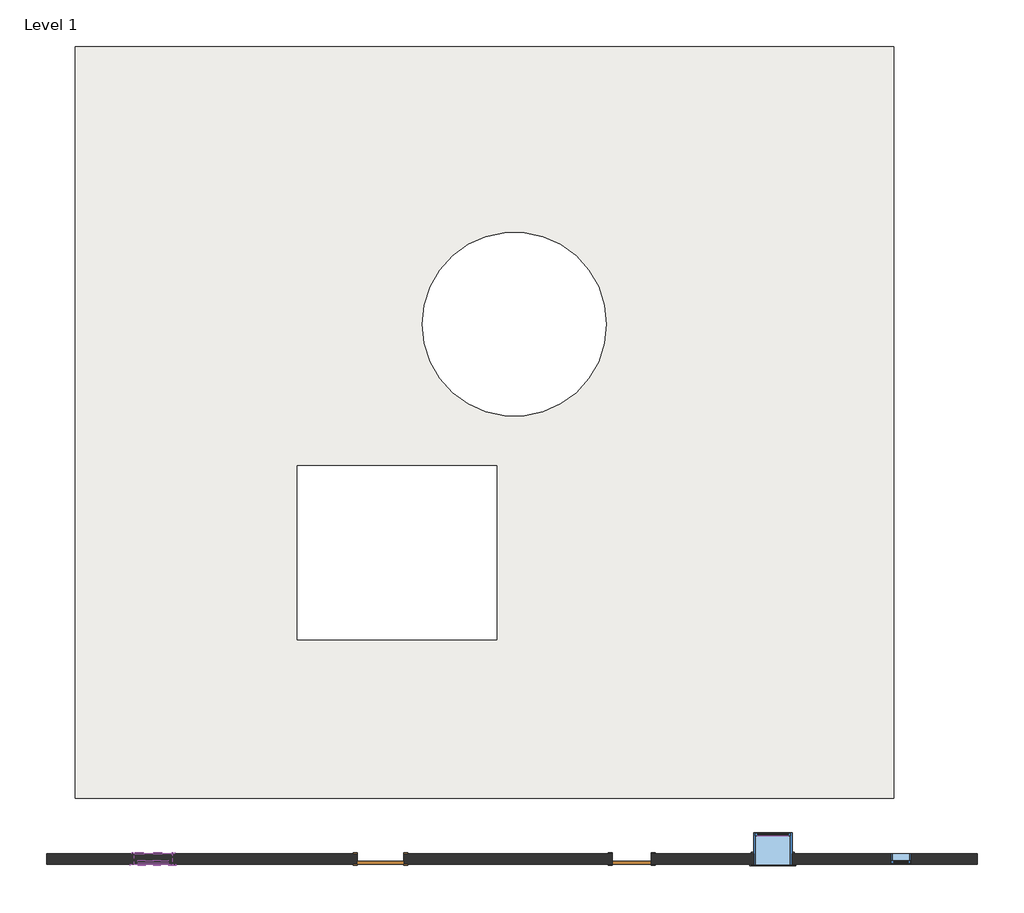
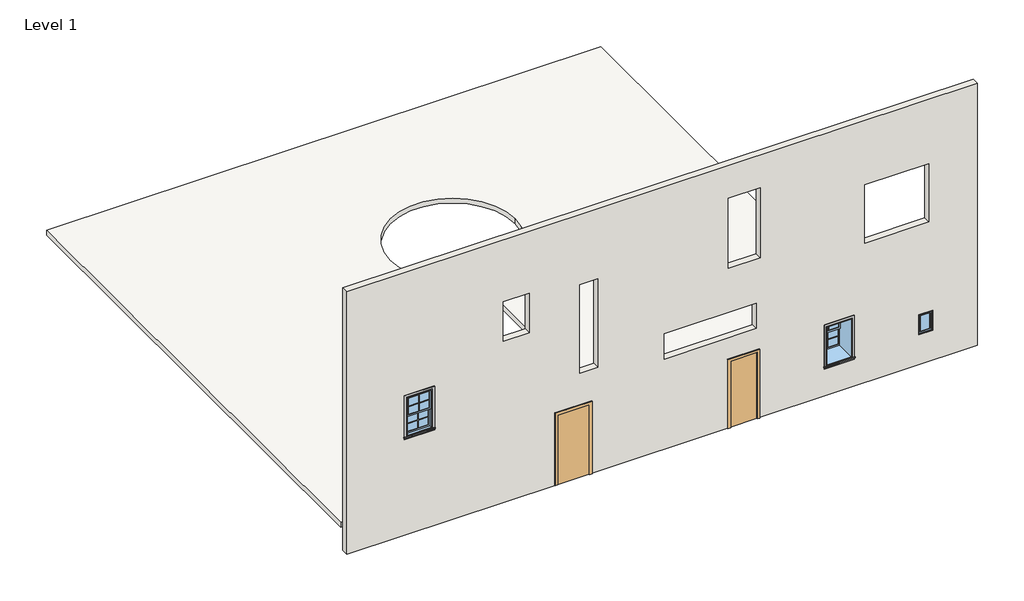
# One storey: 8 proxies, 3 windows, 2 doors, 1 slab, 1 wall.
"""IFC4 building model written with IfcOpenShell, lengths in millimetres."""

import ifcopenshell
import ifcopenshell.guid

model = None  # the IFC model being written
_history = None  # IfcOwnerHistory: only IFC2X3 demands one
_inside = {}  # id of a spatial element -> (the spatial element, [elements in it])
_under = {}  # id of a project, library or spatial element -> (it, [spatial elements below it])
_declared = {}  # id of a project -> (the project, [libraries it declares])
_typed = {}  # id of a type object -> (the type object, [elements of that type])
_made_of = {}  # id of a material, layer set ... -> (it, [elements and type objects made of it])


def new_model(schema):
    """Start an empty IFC model of exactly this schema.

    Asked for "IFC4X3", IfcOpenShell would pick the latest addendum, in which some entities
    have other attributes; the version numbers below select the first issue.
    IFC2X3 requires an IfcOwnerHistory on every rooted entity: one is made here for all.
    """
    global model, _history
    if schema == "IFC4X3":
        model = ifcopenshell.file(schema_version=(4, 3, 0, 0))
    else:
        model = ifcopenshell.file(schema=schema)
    _inside.clear()
    _under.clear()
    _declared.clear()
    _typed.clear()
    _made_of.clear()
    _history = None
    if model.schema == "IFC2X3":
        org = make("IfcOrganization", Name="unknown")
        user = make(
            "IfcPersonAndOrganization",
            ThePerson=make("IfcPerson", FamilyName="unknown"),
            TheOrganization=org,
        )
        app = make(
            "IfcApplication",
            ApplicationDeveloper=org,
            Version="unknown",
            ApplicationFullName="unknown",
            ApplicationIdentifier="unknown",
        )
        _history = make(
            "IfcOwnerHistory",
            OwningUser=user,
            OwningApplication=app,
            ChangeAction="ADDED",
            CreationDate=0,
        )
    return model


def make(cls, **values):
    """One entity of the class cls with the attributes given. An attribute that is None is left unset."""
    return model.create_entity(
        cls, **{name: value for name, value in values.items() if value is not None}
    )


def rooted(cls, **values):
    """An entity with a GlobalId (a new one), such as an element, a storey or a relation."""
    return make(cls, GlobalId=ifcopenshell.guid.new(), OwnerHistory=_history, **values)


def si_unit(unit_type, name, prefix=None):
    """IfcSIUnit, for example si_unit("LENGTHUNIT", "METRE", prefix="MILLI")."""
    return make("IfcSIUnit", UnitType=unit_type, Prefix=prefix, Name=name)


def assignment(units):
    """IfcUnitAssignment: the units of a project."""
    return None if units is None else make("IfcUnitAssignment", Units=units)


def point(xyz):
    """IfcCartesianPoint."""
    return None if xyz is None else make("IfcCartesianPoint", Coordinates=xyz)


def direction(xyz):
    """IfcDirection."""
    return None if xyz is None else make("IfcDirection", DirectionRatios=xyz)


def frame(location, z_axis=None, x_axis=None):
    """IfcAxis2Placement3D, a coordinate frame: its origin and axes. An axis left out is left unset."""
    return make(
        "IfcAxis2Placement3D",
        Location=point(location),
        Axis=direction(z_axis),
        RefDirection=direction(x_axis),
    )


def frame_2d(location, x_axis=None):
    """IfcAxis2Placement2D, a coordinate frame in the plane: its origin and x axis."""
    return make(
        "IfcAxis2Placement2D", Location=point(location), RefDirection=direction(x_axis)
    )


def origin():
    """The frame at (0, 0, 0) with its axes left unset."""
    return frame((0.0, 0.0, 0.0))


def origin_with_axes():
    """The frame at (0, 0, 0) with the z axis (0, 0, 1) and the x axis (1, 0, 0) written out."""
    return frame((0.0, 0.0, 0.0), z_axis=(0.0, 0.0, 1.0), x_axis=(1.0, 0.0, 0.0))


def place(relative_to, where):
    """IfcLocalPlacement: puts the frame where relative to a parent placement (None: the world)."""
    return make(
        "IfcLocalPlacement", PlacementRelTo=relative_to, RelativePlacement=where
    )


def context(
    kind, dimensions, precision=None, world=None, true_north=None, identifier=None
):
    """IfcGeometricRepresentationContext, for example the 3D "Model" context."""
    return make(
        "IfcGeometricRepresentationContext",
        ContextIdentifier=identifier,
        ContextType=kind,
        CoordinateSpaceDimension=dimensions,
        Precision=precision,
        WorldCoordinateSystem=world,
        TrueNorth=true_north,
    )


def project(units=None, contexts=None):
    """IfcProject with its units and contexts."""
    return rooted(
        "IfcProject",
        Name="project",
        RepresentationContexts=contexts,
        UnitsInContext=assignment(units),
    )


def spatial(cls, under=None, at=None, **own):
    """A site, building, storey or space (cls), placed at a placement, below another one or the project."""
    s = rooted(cls, ObjectPlacement=at, **own)
    if under is not None:
        _under.setdefault(under.id(), (under, []))[1].append(s)
    return s


def polyline(points):
    """IfcPolyline through the points."""
    return make("IfcPolyline", Points=[point(p) for p in points])


def circle_curve(where, radius):
    """IfcCircle in the frame where."""
    return make("IfcCircle", Position=where, Radius=radius)


def trimmed(basis, trim1, trim2, sense, master):
    """IfcTrimmedCurve: the piece of a basis curve between two trims."""
    return make(
        "IfcTrimmedCurve",
        BasisCurve=basis,
        Trim1=trim1,
        Trim2=trim2,
        SenseAgreement=sense,
        MasterRepresentation=master,
    )


def segment(curve, same_sense, transition):
    """IfcCompositeCurveSegment."""
    return make(
        "IfcCompositeCurveSegment",
        Transition=transition,
        SameSense=same_sense,
        ParentCurve=curve,
    )


def composite_curve(segments, self_intersect=None):
    """IfcCompositeCurve: segments joined end to end."""
    return make("IfcCompositeCurve", Segments=segments, SelfIntersect=self_intersect)


def outline(outer, holes=None, kind="AREA"):
    """IfcArbitraryClosedProfileDef: a profile drawn as a closed curve; with holes, ...WithVoids."""
    if holes is None:
        return make("IfcArbitraryClosedProfileDef", ProfileType=kind, OuterCurve=outer)
    return make(
        "IfcArbitraryProfileDefWithVoids",
        ProfileType=kind,
        OuterCurve=outer,
        InnerCurves=holes,
    )


def extrude(swept, where, along, depth):
    """IfcExtrudedAreaSolid: the profile swept, set in the frame where, extruded along a direction by depth."""
    return make(
        "IfcExtrudedAreaSolid",
        SweptArea=swept,
        Position=where,
        ExtrudedDirection=direction(along),
        Depth=depth,
    )


def shape(context_of_items, identifier, shape_type, items):
    """IfcShapeRepresentation: the items that make up one representation, for example the "Body"."""
    return make(
        "IfcShapeRepresentation",
        ContextOfItems=context_of_items,
        RepresentationIdentifier=identifier,
        RepresentationType=shape_type,
        Items=items,
    )


def source(mapping_origin, context_of_items, identifier, shape_type, items):
    """IfcRepresentationMap: a shape defined once, which mapped items show again and again."""
    return make(
        "IfcRepresentationMap",
        MappingOrigin=mapping_origin,
        MappedRepresentation=shape(context_of_items, identifier, shape_type, items),
    )


def transform(
    local_origin,
    x_axis=None,
    y_axis=None,
    z_axis=None,
    scale=None,
    scale2=None,
    scale3=None,
    uniform=True,
):
    """IfcCartesianTransformationOperator3D, or its non-uniform kind. x_axis, y_axis, z_axis: its Axis1, 2, 3."""
    if uniform:
        return make(
            "IfcCartesianTransformationOperator3D",
            Axis1=direction(x_axis),
            Axis2=direction(y_axis),
            LocalOrigin=point(local_origin),
            Scale=scale,
            Axis3=direction(z_axis),
        )
    return make(
        "IfcCartesianTransformationOperator3DnonUniform",
        Axis1=direction(x_axis),
        Axis2=direction(y_axis),
        LocalOrigin=point(local_origin),
        Scale=scale,
        Axis3=direction(z_axis),
        Scale2=scale2,
        Scale3=scale3,
    )


def mapped(mapping_source, mapping_target):
    """IfcMappedItem: shows the shape of a source again, moved by a transform."""
    return make(
        "IfcMappedItem", MappingSource=mapping_source, MappingTarget=mapping_target
    )


def made_of(thing, what):
    """Note that an element or type object is made of a material, layer set ...; save() writes the relation."""
    if what is not None:
        _made_of.setdefault(what.id(), (what, []))[1].append(thing)
    return thing


def element(
    cls,
    number,
    at=None,
    inside=None,
    cuts=None,
    type_object=None,
    material=None,
    context=None,
    identifier="Body",
    shape_type=None,
    held_by="IfcProductDefinitionShape",
    body=None,
    shapes=None,
    **own,
):
    """One element of the class cls, such as IfcWall. Its Tag is "e" and its number.

    at: its placement. inside: the storey or other place that contains it. cuts: it is an
    opening in that element (IfcRelVoidsElement). A single representation is given by context,
    identifier, shape_type and body (its items); several are given by shapes. held_by: the class
    of the entity that holds the representations. save() writes the other relations.
    """
    e = rooted(cls, Tag="e%d" % number, ObjectPlacement=at, **own)
    if body is not None:
        shapes = [shape(context, identifier, shape_type, body)]
    if shapes is not None:
        e.Representation = make(held_by, Representations=shapes)
    if inside is not None:
        _inside.setdefault(inside.id(), (inside, []))[1].append(e)
    if cuts is not None:
        rooted(
            "IfcRelVoidsElement", RelatingBuildingElement=cuts, RelatedOpeningElement=e
        )
    if type_object is not None:
        _typed.setdefault(type_object.id(), (type_object, []))[1].append(e)
    return made_of(e, material)


def aggregate(whole, parts):
    """IfcRelAggregates: a whole, such as a stair, and the parts it consists of."""
    return rooted("IfcRelAggregates", RelatingObject=whole, RelatedObjects=parts)


def save(model, path):
    """Write the relations noted so far, then the file.

    IfcRelAggregates (storeys below a building ...), IfcRelContainedInSpatialStructure (elements
    in a storey), IfcRelDefinesByType, IfcRelAssociatesMaterial and IfcRelDeclares: one each for
    every whole, place, type object, material and project.
    """
    for whole, parts in _under.values():
        aggregate(whole, parts)
    for where, things in _inside.values():
        rooted(
            "IfcRelContainedInSpatialStructure",
            RelatedElements=things,
            RelatingStructure=where,
        )
    for kind, things in _typed.values():
        rooted("IfcRelDefinesByType", RelatedObjects=things, RelatingType=kind)
    for what, things in _made_of.values():
        rooted("IfcRelAssociatesMaterial", RelatedObjects=things, RelatingMaterial=what)
    for by, libraries in _declared.values():
        rooted("IfcRelDeclares", RelatingContext=by, RelatedDefinitions=libraries)
    model.write(path)


def m_muntin_pattern_2x2_m_muntin_pattern_2x2_aaec3afb(model_context):
    return source(origin(), model_context, "Body", "SweptSolid", [
        extrude(outline(polyline([(257.1375, -6.35), (257.1375, -298.8), (244.4375, -298.8), (244.4375, -6.35), (0.0, -6.35), (0.0, 6.35), (244.4375, 6.35), (244.4375, 298.8), (257.1375, 298.8), (257.1375, 6.35), (501.575, 6.35), (501.575, -6.35), (257.1375, -6.35)])), frame((0.0, 9.525, 0.0), z_axis=(0.0, 1.0, 0.0), x_axis=(0.0, 0.0, 1.0)), (0.0, 0.0, 1.0), 12.7),
        extrude(outline(polyline([(257.1375, -6.35), (257.1375, -298.8), (244.4375, -298.8), (244.4375, -6.35), (0.0, -6.35), (0.0, 6.35), (244.4375, 6.35), (244.4375, 298.8), (257.1375, 298.8), (257.1375, 6.35), (501.575, 6.35), (501.575, -6.35), (257.1375, -6.35)])), frame((0.0, -22.225, 0.0), z_axis=(0.0, 1.0, 0.0), x_axis=(0.0, 0.0, 1.0)), (0.0, 0.0, 1.0), 12.7),
    ])


def m_trim_window_exterior_flat_with_sill_e7ff6350(model_context):
    return source(origin(), model_context, "Body", "SweptSolid", [
        extrude(outline(polyline([(435.0, -1220.4323709), (435.0, -1280.4323709), (-435.0, -1280.4323709), (-435.0, -1220.4323709), (435.0, -1220.4323709)])), origin_with_axes(), (0.0, 0.0, 1.0), 19.05),
        extrude(outline(polyline([(-1230.0, 38.1), (-1202.4580645, 38.1), (-1200.0, 19.05), (-1200.0, 0.0), (-1220.4323709, 0.0), (-1220.4323709, 19.05), (-1230.0, 19.05), (-1230.0, 38.1)])), frame((-447.7, 0.0, 0.0), z_axis=(1.0, 0.0, 0.0), x_axis=(0.0, 1.0, 0.0)), (0.0, 0.0, 1.0), 895.4),
        extrude(outline(polyline([(-435.0, 60.0), (435.0, 60.0), (435.0, -1200.0), (375.0, -1200.0), (375.0, 0.0), (-375.0, 0.0), (-375.0, -1200.0), (-435.0, -1200.0), (-435.0, 60.0)])), origin_with_axes(), (0.0, 0.0, 1.0), 19.05),
    ])


def m_trim_window_interior_flat_picture_frame_31bd2320(model_context):
    return source(origin(), model_context, "Body", "SweptSolid", [
        extrude(outline(polyline([(422.3, 47.3), (422.3, -1247.3), (-422.3, -1247.3), (-422.3, 47.3), (422.3, 47.3)]), holes=[polyline([(362.3, -12.7), (-362.3, -12.7), (-362.3, -1187.3), (362.3, -1187.3), (362.3, -12.7)])]), origin_with_axes(), (0.0, 0.0, 1.0), 30.0),
    ])


def m_single_flush_0762_x_2032mm_0c256fab(model_context):
    return source(origin(), model_context, "Body", "SweptSolid", [
        extrude(outline(polyline([(2108.0, -457.0), (0.0, -457.0), (0.0, -381.0), (2032.0, -381.0), (2032.0, 381.0), (0.0, 381.0), (0.0, 457.0), (2108.0, 457.0), (2108.0, -457.0)])), frame((0.0, 100.0, 0.0), z_axis=(0.0, 1.0, 0.0), x_axis=(0.0, 0.0, 1.0)), (0.0, 0.0, 1.0), 25.0),
        extrude(outline(polyline([(2108.0, 457.0), (2108.0, -457.0), (0.0, -457.0), (0.0, -381.0), (2032.0, -381.0), (2032.0, 381.0), (0.0, 381.0), (0.0, 457.0), (2108.0, 457.0)])), frame((0.0, -125.0, 0.0), z_axis=(0.0, 1.0, 0.0), x_axis=(0.0, 0.0, 1.0)), (0.0, 0.0, 1.0), 25.0),
        extrude(outline(polyline([(381.0, 49.0), (-381.0, 49.0), (-381.0, 100.0), (381.0, 100.0), (381.0, 49.0)])), origin_with_axes(), (0.0, 0.0, 1.0), 2032.0),
    ])


def m_single_flush_0915_x_2134mm_727434cd(model_context):
    return source(origin(), model_context, "Body", "SweptSolid", [
        extrude(outline(polyline([(2210.0, -533.5), (0.0, -533.5), (0.0, -457.5), (2134.0, -457.5), (2134.0, 457.5), (0.0, 457.5), (0.0, 533.5), (2210.0, 533.5), (2210.0, -533.5)])), frame((0.0, -125.0, 0.0), z_axis=(0.0, 1.0, 0.0), x_axis=(0.0, 0.0, 1.0)), (0.0, 0.0, 1.0), 25.0),
        extrude(outline(polyline([(2210.0, 533.5), (2210.0, -533.5), (0.0, -533.5), (0.0, -457.5), (2134.0, -457.5), (2134.0, 457.5), (0.0, 457.5), (0.0, 533.5), (2210.0, 533.5)])), frame((0.0, 100.0, 0.0), z_axis=(0.0, 1.0, 0.0), x_axis=(0.0, 0.0, 1.0)), (0.0, 0.0, 1.0), 25.0),
        extrude(outline(polyline([(457.5, -49.0), (457.5, -100.0), (-457.5, -100.0), (-457.5, -49.0), (457.5, -49.0)])), origin_with_axes(), (0.0, 0.0, 1.0), 2134.0),
    ])


def m_fixed_0406_x_0610mm_8205b201(model_context):
    return source(origin(), model_context, "Body", "SweptSolid", [
        extrude(outline(polyline([(-140.0, 78.0), (140.0, 78.0), (140.0, 66.0), (-140.0, 66.0), (-140.0, 78.0)])), frame((0.0, 0.0, 978.0), z_axis=(0.0, 0.0, 1.0), x_axis=(1.0, 0.0, 0.0)), (0.0, 0.0, 1.0), 484.0),
        extrude(outline(polyline([(1506.0, -184.0), (934.0, -184.0), (934.0, 184.0), (1506.0, 184.0), (1506.0, -184.0)]), holes=[polyline([(1462.0, -140.0), (1462.0, 140.0), (978.0, 140.0), (978.0, -140.0), (1462.0, -140.0)])]), frame((0.0, 50.0, 0.0), z_axis=(0.0, 1.0, 0.0), x_axis=(0.0, 0.0, 1.0)), (0.0, 0.0, 1.0), 44.0),
        extrude(outline(polyline([(1525.0, -203.0), (915.0, -203.0), (915.0, 203.0), (1525.0, 203.0), (1525.0, -203.0)]), holes=[polyline([(1506.0, -184.0), (1506.0, 184.0), (934.0, 184.0), (934.0, -184.0), (1506.0, -184.0)])]), frame((0.0, 50.0, 0.0), z_axis=(0.0, 1.0, 0.0), x_axis=(0.0, 0.0, 1.0)), (0.0, 0.0, 1.0), 63.0),
        extrude(outline(polyline([(1525.0, -203.0), (915.0, -203.0), (915.0, 203.0), (1525.0, 203.0), (1525.0, -203.0)]), holes=[polyline([(1493.0, -171.0), (1493.0, 171.0), (947.0, 171.0), (947.0, -171.0), (1493.0, -171.0)])]), frame((0.0, -87.0, 0.0), z_axis=(0.0, 1.0, 0.0), x_axis=(0.0, 0.0, 1.0)), (0.0, 0.0, 1.0), 137.0),
    ])


def m_window_double_hung_750_x_1200mm_41070976(model_context):
    return source(origin(), model_context, "Body", "SweptSolid", [
        extrude(outline(polyline([(298.8, 30.15), (298.8, 23.8), (-298.8, 23.8), (-298.8, 30.15), (298.8, 30.15)])), frame((0.0, 0.0, 990.6), z_axis=(0.0, 0.0, 1.0), x_axis=(1.0, 0.0, 0.0)), (0.0, 0.0, 1.0), 501.575),
        extrude(outline(polyline([(-298.8, 17.45), (298.8, 17.45), (298.8, 11.1), (-298.8, 11.1), (-298.8, 17.45)])), frame((0.0, 0.0, 990.6), z_axis=(0.0, 0.0, 1.0), x_axis=(1.0, 0.0, 0.0)), (0.0, 0.0, 1.0), 501.575),
        extrude(outline(polyline([(298.8, 74.6), (298.8, 68.25), (-298.8, 68.25), (-298.8, 74.6), (298.8, 74.6)])), frame((0.0, 0.0, 1536.625), z_axis=(0.0, 0.0, 1.0), x_axis=(1.0, 0.0, 0.0)), (0.0, 0.0, 1.0), 501.575),
        extrude(outline(polyline([(-298.8, 61.9), (298.8, 61.9), (298.8, 55.55), (-298.8, 55.55), (-298.8, 61.9)])), frame((0.0, 0.0, 1536.625), z_axis=(0.0, 0.0, 1.0), x_axis=(1.0, 0.0, 0.0)), (0.0, 0.0, 1.0), 501.575),
        extrude(outline(polyline([(1536.625, -343.25), (946.15, -343.25), (946.15, 343.25), (1536.625, 343.25), (1536.625, -343.25)]), holes=[polyline([(1492.175, 298.8), (990.6, 298.8), (990.6, -298.8), (1492.175, -298.8), (1492.175, 298.8)])]), frame((0.0, -1.6, 0.0), z_axis=(0.0, 1.0, 0.0), x_axis=(0.0, 0.0, 1.0)), (0.0, 0.0, 1.0), 44.45),
        extrude(outline(polyline([(2082.65, -343.25), (1492.175, -343.25), (1492.175, 343.25), (2082.65, 343.25), (2082.65, -343.25)]), holes=[polyline([(2038.2, 298.8), (1536.625, 298.8), (1536.625, -298.8), (2038.2, -298.8), (2038.2, 298.8)])]), frame((0.0, 42.85, 0.0), z_axis=(0.0, 1.0, 0.0), x_axis=(0.0, 0.0, 1.0)), (0.0, 0.0, 1.0), 44.45),
        extrude(outline(polyline([(2114.4, -375.0), (914.4, -375.0), (914.4, 375.0), (2114.4, 375.0), (2114.4, -375.0)]), holes=[polyline([(2082.65, 343.25), (946.15, 343.25), (946.15, -343.25), (2082.65, -343.25), (2082.65, 343.25)])]), frame((0.0, -14.3, 0.0), z_axis=(0.0, 1.0, 0.0), x_axis=(0.0, 0.0, 1.0)), (0.0, 0.0, 1.0), 133.35),
        extrude(outline(polyline([(2114.4, 375.0), (2114.4, -375.0), (914.4, -375.0), (914.4, 375.0), (2114.4, 375.0)]), holes=[polyline([(2095.35, 355.95), (933.45, 355.95), (933.45, -355.95), (2095.35, -355.95), (2095.35, 355.95)])]), frame((0.0, -100.0, 0.0), z_axis=(0.0, 1.0, 0.0), x_axis=(0.0, 0.0, 1.0)), (0.0, 0.0, 1.0), 85.7),
    ])


def m_window_double_hung_750_x_1200mm_e21ea802(model_context):
    return source(origin(), model_context, "Body", "SweptSolid", [
        extrude(outline(polyline([(298.8, -469.85), (298.8, -476.2), (-298.8, -476.2), (-298.8, -469.85), (298.8, -469.85)])), frame((0.0, 0.0, 990.6), z_axis=(0.0, 0.0, 1.0), x_axis=(1.0, 0.0, 0.0)), (0.0, 0.0, 1.0), 501.575),
        extrude(outline(polyline([(-298.8, -482.55), (298.8, -482.55), (298.8, -488.9), (-298.8, -488.9), (-298.8, -482.55)])), frame((0.0, 0.0, 990.6), z_axis=(0.0, 0.0, 1.0), x_axis=(1.0, 0.0, 0.0)), (0.0, 0.0, 1.0), 501.575),
        extrude(outline(polyline([(298.8, -425.4), (298.8, -431.75), (-298.8, -431.75), (-298.8, -425.4), (298.8, -425.4)])), frame((0.0, 0.0, 1536.625), z_axis=(0.0, 0.0, 1.0), x_axis=(1.0, 0.0, 0.0)), (0.0, 0.0, 1.0), 501.575),
        extrude(outline(polyline([(-298.8, -438.1), (298.8, -438.1), (298.8, -444.45), (-298.8, -444.45), (-298.8, -438.1)])), frame((0.0, 0.0, 1536.625), z_axis=(0.0, 0.0, 1.0), x_axis=(1.0, 0.0, 0.0)), (0.0, 0.0, 1.0), 501.575),
        extrude(outline(polyline([(1536.625, -343.25), (946.15, -343.25), (946.15, 343.25), (1536.625, 343.25), (1536.625, -343.25)]), holes=[polyline([(1492.175, 298.8), (990.6, 298.8), (990.6, -298.8), (1492.175, -298.8), (1492.175, 298.8)])]), frame((0.0, -501.6, 0.0), z_axis=(0.0, 1.0, 0.0), x_axis=(0.0, 0.0, 1.0)), (0.0, 0.0, 1.0), 44.45),
        extrude(outline(polyline([(2082.65, -343.25), (1492.175, -343.25), (1492.175, 343.25), (2082.65, 343.25), (2082.65, -343.25)]), holes=[polyline([(2038.2, 298.8), (1536.625, 298.8), (1536.625, -298.8), (2038.2, -298.8), (2038.2, 298.8)])]), frame((0.0, -457.15, 0.0), z_axis=(0.0, 1.0, 0.0), x_axis=(0.0, 0.0, 1.0)), (0.0, 0.0, 1.0), 44.45),
        extrude(outline(polyline([(2114.4, -375.0), (914.4, -375.0), (914.4, 375.0), (2114.4, 375.0), (2114.4, -375.0)]), holes=[polyline([(2082.65, 343.25), (946.15, 343.25), (946.15, -343.25), (2082.65, -343.25), (2082.65, 343.25)])]), frame((0.0, -514.3, 0.0), z_axis=(0.0, 1.0, 0.0), x_axis=(0.0, 0.0, 1.0)), (0.0, 0.0, 1.0), 633.35),
    ])


model = new_model("IFC4")

# Units and contexts
model_context = context("Model", 3, world=origin())
ifc_project = project(units=[si_unit("LENGTHUNIT", "METRE", prefix="MILLI")], contexts=[model_context])

# Site, building, storey
site = spatial("IfcSite", under=ifc_project)
building = spatial("IfcBuilding", under=site)
storey = spatial("IfcBuildingStorey", under=building, Name="Level 1", Elevation=0.0)

# Proxies
placement = place(None, origin())
m_muntin_pattern_2x2_m_muntin_pattern_2x2_shape = m_muntin_pattern_2x2_m_muntin_pattern_2x2_aaec3afb(model_context)
element("IfcBuildingElementProxy", 1, Name="M_Muntin Pattern_2x2 : M_Muntin Pattern_2x2", ObjectType="M_Muntin Pattern_2x2 : M_Muntin Pattern_2x2", at=placement, inside=storey, context=model_context, shape_type="MappedRepresentation", body=[
    mapped(m_muntin_pattern_2x2_m_muntin_pattern_2x2_shape, transform((-9517.9287267, -12044.9889904, 3622.225), x_axis=(-1.0, 0.0, 0.0), y_axis=(0.0, -1.0, 0.0), z_axis=(0.0, 0.0, 1.0))),
])
element("IfcBuildingElementProxy", 2, Name="M_Muntin Pattern_2x2 : M_Muntin Pattern_2x2", ObjectType="M_Muntin Pattern_2x2 : M_Muntin Pattern_2x2", at=placement, inside=storey, context=model_context, shape_type="MappedRepresentation", body=[
    mapped(m_muntin_pattern_2x2_m_muntin_pattern_2x2_shape, transform((-9517.9287267, -12000.5389904, 3076.2), x_axis=(-1.0, 0.0, 0.0), y_axis=(0.0, -1.0, 0.0), z_axis=(0.0, 0.0, 1.0))),
])
element("IfcBuildingElementProxy", 3, Name="M_Muntin Pattern_2x2 : M_Muntin Pattern_2x2", ObjectType="M_Muntin Pattern_2x2 : M_Muntin Pattern_2x2", at=placement, inside=storey, context=model_context, shape_type="MappedRepresentation", body=[
    mapped(m_muntin_pattern_2x2_m_muntin_pattern_2x2_shape, transform((2597.0712733, -11544.9889904, 1536.625), x_axis=(-1.0, 0.0, 0.0), y_axis=(0.0, -1.0, 0.0), z_axis=(0.0, 0.0, 1.0))),
])
element("IfcBuildingElementProxy", 4, Name="M_Muntin Pattern_2x2 : M_Muntin Pattern_2x2", ObjectType="M_Muntin Pattern_2x2 : M_Muntin Pattern_2x2", at=placement, inside=storey, context=model_context, shape_type="MappedRepresentation", body=[
    mapped(m_muntin_pattern_2x2_m_muntin_pattern_2x2_shape, transform((2597.0712733, -11500.5389904, 990.6), x_axis=(-1.0, 0.0, 0.0), y_axis=(0.0, -1.0, 0.0), z_axis=(0.0, 0.0, 1.0))),
])
m_trim_window_exterior_flat_with_sill_shape = m_trim_window_exterior_flat_with_sill_e7ff6350(model_context)
element("IfcBuildingElementProxy", 5, Name="M_Trim-Window-Exterior-Flat : with Sill", ObjectType="M_Trim-Window-Exterior-Flat : with Sill", at=placement, inside=storey, context=model_context, shape_type="MappedRepresentation", body=[
    mapped(m_trim_window_exterior_flat_with_sill_shape, transform((-9517.9287267, -12079.9139904, 4200.0), x_axis=(1.0, 0.0, 0.0), y_axis=(0.0, 0.0, 1.0), z_axis=(0.0, -1.0, 0.0))),
])
element("IfcBuildingElementProxy", 6, Name="M_Trim-Window-Exterior-Flat : with Sill", ObjectType="M_Trim-Window-Exterior-Flat : with Sill", at=placement, inside=storey, context=model_context, shape_type="MappedRepresentation", body=[
    mapped(m_trim_window_exterior_flat_with_sill_shape, transform((2597.0712733, -12079.9139904, 2114.4), x_axis=(1.0, 0.0, 0.0), y_axis=(0.0, 0.0, 1.0), z_axis=(0.0, -1.0, 0.0))),
])
m_trim_window_interior_flat_picture_frame_shape = m_trim_window_interior_flat_picture_frame_31bd2320(model_context)
element("IfcBuildingElementProxy", 7, Name="M_Trim-Window-Interior-Flat : Picture Frame", ObjectType="M_Trim-Window-Interior-Flat : Picture Frame", at=placement, inside=storey, context=model_context, shape_type="MappedRepresentation", body=[
    mapped(m_trim_window_interior_flat_picture_frame_shape, transform((-9517.9287267, -11879.9139904, 4200.0), x_axis=(-1.0, 0.0, 0.0), y_axis=(0.0, 0.0, 1.0), z_axis=(0.0, 1.0, 0.0))),
])
element("IfcBuildingElementProxy", 8, Name="M_Trim-Window-Interior-Flat : Picture Frame", ObjectType="M_Trim-Window-Interior-Flat : Picture Frame", at=placement, inside=storey, context=model_context, shape_type="MappedRepresentation", body=[
    mapped(m_trim_window_interior_flat_picture_frame_shape, transform((2597.0712733, -11879.9139904, 2114.4), x_axis=(-1.0, 0.0, 0.0), y_axis=(0.0, 0.0, 1.0), z_axis=(0.0, 1.0, 0.0))),
])

# Doors
m_single_flush_0762_x_2032mm_shape = m_single_flush_0762_x_2032mm_0c256fab(model_context)
element("IfcDoor", 9, ObjectType="M_Single-Flush : 0762 x 2032mm", at=placement, inside=storey, context=model_context, shape_type="MappedRepresentation", body=[
    mapped(m_single_flush_0762_x_2032mm_shape, transform((-160.4287267, -11979.9139904, 0.0), x_axis=(-1.0, 0.0, 0.0), y_axis=(0.0, -1.0, 0.0), z_axis=(0.0, 0.0, 1.0))),
])
m_single_flush_0915_x_2134mm_shape = m_single_flush_0915_x_2134mm_727434cd(model_context)
element("IfcDoor", 10, ObjectType="M_Single-Flush : 0915 x 2134mm", at=placement, inside=storey, context=model_context, shape_type="MappedRepresentation", body=[
    mapped(m_single_flush_0915_x_2134mm_shape, transform((-5075.4287267, -11979.9139904, 0.0), x_axis=(1.0, 0.0, 0.0), y_axis=(0.0, 1.0, 0.0), z_axis=(0.0, 0.0, 1.0))),
])

# Slab
element("IfcSlab", 11, ObjectType="Generic 150mm", at=placement, inside=storey, context=model_context, shape_type="SweptSolid", body=[
    extrude(outline(polyline([(4955.9656102, -10797.4121597), (-11044.0343898, -10797.4121597), (-11044.0343898, 3902.5878403), (4955.9656102, 3902.5878403), (4955.9656102, -10797.4121597)]), holes=[polyline([(-2803.5612558, -7694.4830059), (-2803.5612558, -4294.4830059), (-6703.5612558, -4294.4830059), (-6703.5612558, -7694.4830059), (-2803.5612558, -7694.4830059)]), composite_curve([segment(trimmed(circle_curve(frame_2d((-2455.6131826, -1525.5713844)), 1800.0), [point((-4255.6131826, -1525.5713844))], [point((-655.6131826, -1525.5713844))], True, "CARTESIAN"), True, "CONTINUOUS"), segment(trimmed(circle_curve(frame_2d((-2455.6131826, -1525.5713844)), 1800.0), [point((-655.6131826, -1525.5713844))], [point((-4255.6131826, -1525.5713844))], True, "CARTESIAN"), True, "CONTINUOUS")], self_intersect=False)]), frame((0.0, 0.0, -150.0), z_axis=(0.0, 0.0, 1.0), x_axis=(1.0, 0.0, 0.0)), (0.0, 0.0, 1.0), 150.0),
])

# Wall
element("IfcWall", 12, ObjectType="Generic - 200mm", at=placement, inside=storey, context=model_context, shape_type="SweptSolid", body=[
    extrude(outline(polyline([(0.0, 6597.0712733), (8000.0, 6597.0712733), (8000.0, -11602.9287267), (0.0, -11602.9287267), (0.0, -5532.9287267), (2134.0, -5532.9287267), (2134.0, -4617.9287267), (0.0, -4617.9287267), (0.0, -541.4287267), (2032.0, -541.4287267), (2032.0, 220.5712733), (0.0, 220.5712733), (0.0, 6597.0712733)]), holes=[polyline([(915.0, 5303.0712733), (915.0, 4897.0712733), (1525.0, 4897.0712733), (1525.0, 5303.0712733), (915.0, 5303.0712733)]), polyline([(2114.4, 2972.0712733), (914.4, 2972.0712733), (914.4, 2222.0712733), (2114.4, 2222.0712733), (2114.4, 2972.0712733)]), polyline([(4200.0, -9142.9287267), (3000.0, -9142.9287267), (3000.0, -9892.9287267), (4200.0, -9892.9287267), (4200.0, -9142.9287267)]), polyline([(6114.4, -6332.9287267), (4914.4, -6332.9287267), (4914.4, -7082.9287267), (6114.4, -7082.9287267), (6114.4, -6332.9287267)]), polyline([(4866.0, -592.9287267), (7000.0, -592.9287267), (7000.0, 322.0712733), (4866.0, 322.0712733), (4866.0, -592.9287267)]), polyline([(5863.7369526, -4875.7403935), (5863.7369526, -4355.210627), (3168.8098281, -4355.210627), (3168.8098281, -4875.7403935), (5863.7369526, -4875.7403935)]), polyline([(3522.0583984, -2446.6014834), (3522.0583984, 213.8839896), (2748.6051294, 213.8839896), (2748.6051294, -2446.6014834), (3522.0583984, -2446.6014834)]), polyline([(6036.9886823, 3337.0625883), (6036.9886823, 5187.8350912), (4260.1064286, 5187.8350912), (4260.1064286, 3337.0625883), (6036.9886823, 3337.0625883)])]), frame((0.0, -12079.9139904, 0.0), z_axis=(0.0, 1.0, 0.0), x_axis=(0.0, 0.0, 1.0)), (0.0, 0.0, 1.0), 200.0),
])

# Windows
m_fixed_0406_x_0610mm_shape = m_fixed_0406_x_0610mm_8205b201(model_context)
element("IfcWindow", 13, ObjectType="M_Fixed : 0406 x 0610mm", at=placement, inside=storey, context=model_context, shape_type="MappedRepresentation", body=[
    mapped(m_fixed_0406_x_0610mm_shape, transform((5100.0712733, -11966.9139904, 0.0), x_axis=(-1.0, 0.0, 0.0), y_axis=(0.0, -1.0, 0.0), z_axis=(0.0, 0.0, 1.0))),
])
m_window_double_hung_750_x_1200mm_shape = m_window_double_hung_750_x_1200mm_41070976(model_context)
element("IfcWindow", 14, ObjectType="M_Window-Double-Hung : 750 x 1200mm", at=placement, inside=storey, context=model_context, shape_type="MappedRepresentation", body=[
    mapped(m_window_double_hung_750_x_1200mm_shape, transform((-9517.9287267, -11979.9139904, 2085.6), x_axis=(-1.0, 0.0, 0.0), y_axis=(0.0, -1.0, 0.0), z_axis=(0.0, 0.0, 1.0))),
])
m_window_double_hung_750_x_1200mm_2_shape = m_window_double_hung_750_x_1200mm_e21ea802(model_context)
element("IfcWindow", 15, ObjectType="M_Window-Double-Hung : 750 x 1200mm", at=placement, inside=storey, context=model_context, shape_type="MappedRepresentation", body=[
    mapped(m_window_double_hung_750_x_1200mm_2_shape, transform((2597.0712733, -11979.9139904, 0.0), x_axis=(-1.0, 0.0, 0.0), y_axis=(0.0, -1.0, 0.0), z_axis=(0.0, 0.0, 1.0))),
])

save(model, "model.ifc")

# Revit data of these elements
# Project information
#   Project Issue Date = "Issue Date"
#   Project Status = "Project Status"
#   Client Name = "Owner"
#   Project Address = "Enter address here"
#   Project Name = "Project Name"
#   Project Number = "0001"
# Type "M_Muntin Pattern_2x2 : M_Muntin Pattern_2x2"
#   Width [instance default] = 1200 mm
#   Thickness = 12.7 mm
#   Height [instance default] = 1200 mm
#   Distance = 19.05 mm
#   Interior Material [instance default] = none
#   Exterior Material [instance default] = none
#   Default Elevation = 0
# Type "M_Trim-Window-Exterior-Flat : with Sill"
#   Trim Width = 60 mm
#   Trim Thickness_Picture Frame = 30 mm
#   Trim Thickness_with Sill = 19.05 mm
#   Sill Thickness = 30 mm
#   Opening Width [instance default] = 600 mm
#   Opening Height [instance default] = 900 mm
#   Default Elevation = 1200 mm
#   Sill = yes
#   Picture Frame = no
#   Trim Material [instance default] = none
# Type "M_Trim-Window-Interior-Flat : Picture Frame"
#   Trim Thickness_Picture Frame = 30 mm
#   Trim Width = 60 mm
#   Trim Thickness_with Sill = 20 mm
#   Sill Thickness = 30 mm
#   Opening Width [instance default] = 600 mm
#   Opening Height [instance default] = 900 mm
#   Default Elevation = 1200 mm
#   Sill = no
#   Picture Frame = yes
#   Trim Material [instance default] = none
# Type "M_Single-Flush : 0762 x 2032mm"
#   Type Mark = "28"
#   Construction Type Id = "MDOOR"
#   Analytic Construction = "Metal"
#   Thickness = 51 mm
#   Thermal Resistance (R) = 0.270117 (m²·K)/W
#   Heat Transfer Coefficient (U) = 3.7021 W/(m²·K)
#   Height = 2032 mm
#   Trim Projection Ext = 25 mm
#   Trim Projection Int = 25 mm
#   Trim Width = 76 mm
#   Width = 762 mm
#   Define Thermal Properties by = 1
#   Define Thermal Properties by = 1
#   Door Material = Door - Panel
#   Frame Material = Door - Frame
#   Visual Light Transmittance = 0
#   Solar Heat Gain Coefficient = 0
#   Function = (empty or 0)
#   Wall Closure = (empty or 0)
# Type "M_Single-Flush : 0915 x 2134mm"
#   Type Mark = "20"
#   Construction Type Id = "MDOOR"
#   Analytic Construction = "Metal"
#   Thickness = 51 mm
#   Thermal Resistance (R) = 0.270117 (m²·K)/W
#   Heat Transfer Coefficient (U) = 3.7021 W/(m²·K)
#   Height = 2134 mm
#   Trim Projection Ext = 25 mm
#   Trim Projection Int = 25 mm
#   Trim Width = 76 mm
#   Width = 915 mm
#   Define Thermal Properties by = 1
#   Define Thermal Properties by = 1
#   Door Material = Door - Panel
#   Frame Material = Door - Frame
#   Visual Light Transmittance = 0
#   Solar Heat Gain Coefficient = 0
#   Function = (empty or 0)
#   Wall Closure = (empty or 0)
# Type "Generic 150mm"
#   Function = 0
#   Layers, outside or top first: 150 mm no material (function 1)
# Type "Generic - 200mm"
#   Layers, outside or top first: 200 mm no material (function 1)
# Type "M_Fixed : 0406 x 0610mm"
#   Type Mark = "10"
#   Construction Type Id = "GSP4R"
#   Analytic Construction = "1/8 in Pilkington single glazing"
#   Visual Light Transmittance = 0.9
#   Thermal Resistance (R) = 0.271106 (m²·K)/W
#   Solar Heat Gain Coefficient = 0.78
#   Heat Transfer Coefficient (U) = 3.6886 W/(m²·K)
#   Height = 610 mm
#   Default Sill Height = 915 mm
#   Width = 406 mm
#   Window Inset = 19 mm
#   Define Thermal Properties by = 1
#   Define Thermal Properties by = 1
#   Frame Exterior Material = Sash
#   Frame Interior Material = Sash
#   Glass Pane Material = Glass
#   Sash = Sash
#   Wall Closure = (empty or 0)
# Type "M_Window-Double-Hung : 750 x 1200mm"
#   Type Mark = "22"
#   Fire Rating = "0.5h"
#   Construction Type Id = "DG-DR"
#   Assembly Code = "B2020100"
#   Analytic Construction = "Double glazing - domestic"
#   Wall Thickness [instance default] = 150 mm
#   Window Inset [instance default] = 0 mm
#   Visual Light Transmittance = 0.81
#   Thermal Resistance (R) = 0.319569 (m²·K)/W
#   Solar Heat Gain Coefficient = 0.76
#   Muntin Width = 597.6 mm
#   Muntin Height = 501.575 mm
#   Interior Wall Closure [instance default] = 35.7 mm
#   Rough Width = 765 mm
#   Rough Height = 1215 mm
#   Frame Extension [instance default] = 31.75 mm
#   Exterior Wall Closure [instance default] = 12.7 mm
#   Extension Jamb [instance default] = 35.7 mm
#   Heat Transfer Coefficient (U) = 3.12929 W/(m²·K)
#   Height = 1200 mm
#   Width = 750 mm
#   Define Thermal Properties by = 1
#   Top Muntin Visibility = yes
#   Indicator Visibility [instance default] = yes
#   Extension Jamb Visibility [instance default] = yes
#   Interior Trim Visibility [instance default] = yes
#   Exterior Trim Visibility [instance default] = yes
#   Define Thermal Properties by = 1
#   Bottom Muntin Visibility = yes
#   Muntin Pattern = M_Muntin Pattern_2x2 : M_Muntin Pattern_2x2
#   Interior Trim Material = Wood - Stained
#   Interior Trim = M_Trim-Window-Interior-Flat : Picture Frame
#   Exterior Trim Material = Clad - White
#   Exterior Trim = M_Trim-Window-Exterior-Flat : with Sill
#   Glass Panel Material = Glass
#   Exterior Frame Material = Clad - White
#   Interior Frame Material = Wood - Stained
#   Wall Closure = (empty or 0)
# Elements 1, 2, 3, 4 (IfcBuildingElementProxy, "M_Muntin Pattern_2x2 : M_Muntin Pattern_2x2")
#   Width = 597.6 mm
#   Height = 501.575 mm
#   Interior Material = Wood - Stained
#   Exterior Material = Clad - White
#   Phase Created = New Construction
#   Materials on its faces: "Clad - White", "Wood - Stained"
# Elements 5, 6 (IfcBuildingElementProxy, "M_Trim-Window-Exterior-Flat : with Sill")
#   Opening Width = 750 mm
#   Opening Height = 1200 mm
#   Trim Material = Clad - White
#   Phase Created = New Construction
#   Materials on its faces: "Clad - White"
# Elements 7, 8 (IfcBuildingElementProxy, "M_Trim-Window-Interior-Flat : Picture Frame")
#   Opening Width = 750 mm
#   Opening Height = 1200 mm
#   Trim Material = Wood - Stained
#   Phase Created = New Construction
#   Materials on its faces: "Wood - Stained"
# Element 9 (IfcDoor, "M_Single-Flush : 0762 x 2032mm")
#   Phase Created = New Construction
#   Materials on its faces: "Door - Frame", "Door - Panel"
# Element 10 (IfcDoor, "M_Single-Flush : 0915 x 2134mm")
#   Phase Created = New Construction
#   Materials on its faces: "Door - Frame", "Door - Panel"
# Element 11 (IfcSlab, "Generic 150mm")
#   Height Offset From Level = 0 mm
#   Phase Created = New Construction
#   Materials on its faces: "Default Floor"
# Element 12 (IfcWall, "Generic - 200mm")
#   Top Offset = 0 mm
#   Base Offset = 0 mm
#   Unconnected Height = 8000 mm
#   wall height = 8000 mm
#   Phase Created = New Construction
#   Base Constraint = Level 1
#   Materials on its faces: "Default Wall"
# Element 13 (IfcWindow, "M_Fixed : 0406 x 0610mm")
#   Mark = "1"
#   Phase Created = New Construction
#   Materials on its faces: "Sash", "Glass"
# Element 14 (IfcWindow, "M_Window-Double-Hung : 750 x 1200mm")
#   Mark = "2"
#   Window Inset = 0 mm
#   Interior Wall Closure = 35.7 mm
#   Frame Extension = 31.75 mm
#   Exterior Wall Closure = 12.7 mm
#   Interior Trim Visibility = yes
#   Indicator Visibility = yes
#   Exterior Trim Visibility = yes
#   Phase Created = New Construction
#   Materials on its faces: "Wood - Stained", "Glass", "Clad - White"
# Element 15 (IfcWindow, "M_Window-Double-Hung : 750 x 1200mm")
#   Mark = "3"
#   Window Inset = 500 mm
#   Interior Wall Closure = 35.7 mm
#   Frame Extension = 531.75 mm
#   Exterior Wall Closure = 12.7 mm
#   Interior Trim Visibility = yes
#   Indicator Visibility = yes
#   Exterior Trim Visibility = yes
#   Phase Created = New Construction
#   Materials on its faces: "Wood - Stained", "Glass", "Clad - White"
# Materials
#   "Door - Panel": class "Wood", colour RGB 210 159 95, transparency 0, Cost = 0
#   "Door - Frame": class "Miscellaneous", colour RGB 118 70 51, transparency 0, Cost = 0
#   "Sash": class "Wood", colour RGB 224 178 126, transparency 0, Cost = 0
#   "Glass": class "Glass", colour RGB 0 128 192, transparency 0.9, Description = "Soda Lime Glass", Cost = 0
#   "Wood - Stained": class "Wood", colour RGB 224 178 126, transparency 0, Cost = 0
#   "Clad - White": class "Wood", colour RGB 242 242 238, transparency 0, Cost = 0
#   "Default Floor": class "Miscellaneous", colour RGB 127 127 127, transparency 0, Cost = 0
#   "Default Wall": class "Miscellaneous", colour RGB 128 128 128, transparency 0, Cost = 0
